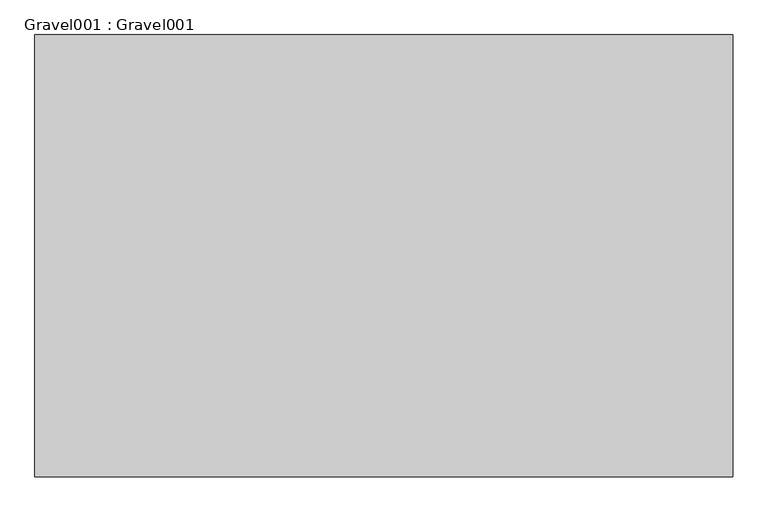
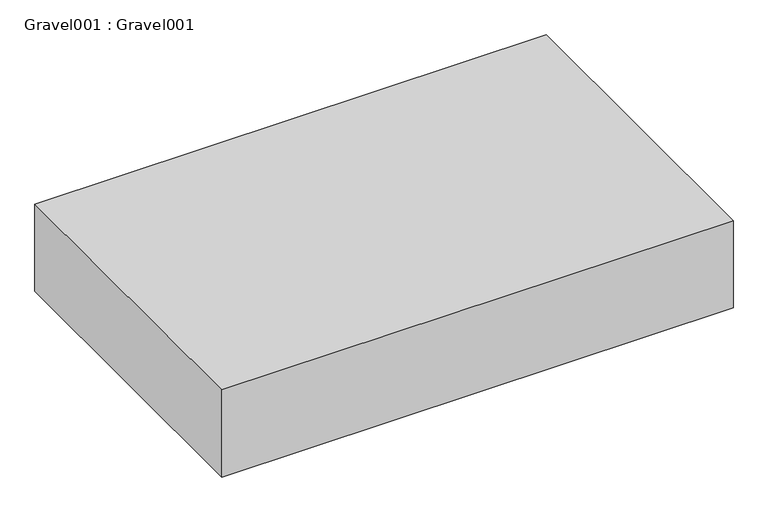
"""IFC4 building model written with IfcOpenShell, lengths in millimetres: proxy geometry, Gravel001 : Gravel001."""

from ifc_helpers import new_model, si_unit, frame, origin, place, context, project, spatial, polyline, outline, extrude, source, transform, mapped, element, save


def gravel001_gravel001_b8bdd5c4(model_context):
    return source(origin(), model_context, "Body", "SweptSolid", [
        extrude(outline(polyline([(14383.0178845, -4637.5417972), (14383.0178845, -5904.2981766), (12383.0178845, -5904.2981766), (12383.0178845, -4637.5417972), (14383.0178845, -4637.5417972)])), frame((0.0, 0.0, 35744.9946418), z_axis=(0.0, 0.0, 1.0), x_axis=(1.0, 0.0, 0.0)), (0.0, 0.0, 1.0), 360.4577188),
    ])


if __name__ == "__main__":
    model = new_model("IFC4")
    model_context = context("Model", 3, world=origin())
    ifc_project = project(units=[si_unit("LENGTHUNIT", "METRE", prefix="MILLI")], contexts=[model_context])
    site = spatial("IfcSite", under=ifc_project)
    building = spatial("IfcBuilding", under=site)
    placement = place(None, origin())
    gravel001_gravel001_shape = gravel001_gravel001_b8bdd5c4(model_context)
    element("IfcBuildingElementProxy", 1, Name="Gravel001 : Gravel001", ObjectType="Gravel001 : Gravel001", at=placement, inside=building, context=model_context, shape_type="MappedRepresentation", body=[
        mapped(gravel001_gravel001_shape, transform((0.0, 0.0, 0.0), x_axis=(1.0, 0.0, 0.0), y_axis=(0.0, 1.0, 0.0), z_axis=(0.0, 0.0, 1.0))),
    ])
    save(model, "model.ifc")

# Revit data of these elements
# Type "Gravel001 : Gravel001"
#   NameOverride = "Gravel001"
# Element 1 (IfcBuildingElementProxy, "Gravel001 : Gravel001")
#   Materials on its faces: "4\" MIN. CRUSHED GRAVEL (NO FINES)"
# Materials
#   "4\" MIN. CRUSHED GRAVEL (NO FINES)": class "Unassigned", colour RGB 145 162 188, transparency 0, Cost = 0
